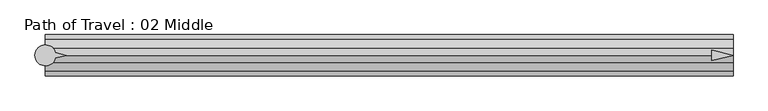
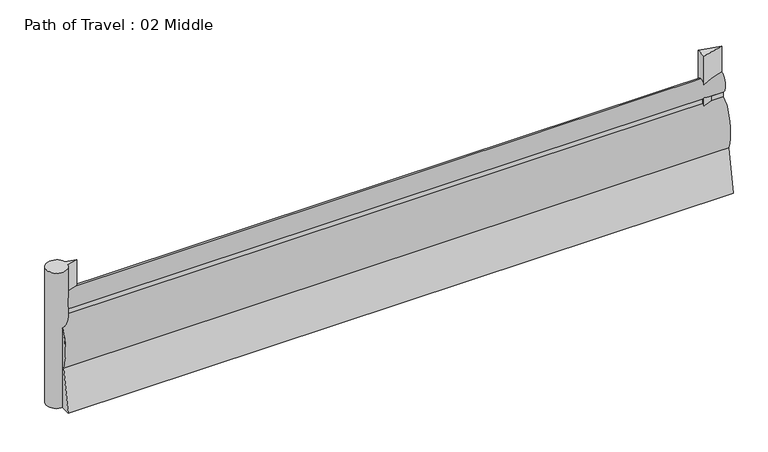
"""IFC4 building model written with IfcOpenShell, lengths in millimetres: proxy geometry, Path of Travel : 02 Middle."""

from ifc_helpers import new_model, si_unit, point, frame, frame_2d, origin, origin_with_axes, place, context, project, spatial, polyline, circle_curve, ellipse_curve, trimmed, segment, composite_curve, outline, extrude, source, transform, mapped, element, save
from ifc_brep_helpers import plane_surface, extruded_surface, advanced_brep


def path_of_travel_02_middle_d07484ce(model_context):
    return source(origin(), model_context, "Body", "SolidModel", [
        advanced_brep(
        [(227.5554837, 0.0, 1727.2), (227.5554837, 42.9018657, 1436.6534209), (227.5554837, 42.9018657, 1363.4763406), (227.5554837, 184.1186263, 643.4144547), (227.5554837, 297.5699544, 0.0), (227.5554837, 145.6574193, 0.0), (227.5554837, 0.0, 584.2), (227.5554837, -145.6574193, 0.0), (227.5554837, -297.5699544, 0.0), (227.5554837, -184.1186263, 643.4144547), (227.5554837, -42.9018657, 1363.4763406), (227.5554837, -42.9018657, 1436.6534209), (10133.5554837, 0.0, 1727.2), (10133.5554837, -42.9018657, 1436.6534209), (10133.5554837, -42.9018657, 1363.4763406), (10133.5554837, -184.1186263, 643.4144547), (10133.5554837, -297.5699544, 0.0), (10133.5554837, -145.6574193, 0.0), (10133.5554837, 0.0, 584.2), (10133.5554837, 145.6574193, 0.0), (10133.5554837, 297.5699544, 0.0), (10133.5554837, 184.1186263, 643.4144547), (10133.5554837, 42.9018657, 1363.4763406), (10133.5554837, 42.9018657, 1436.6534209)],
        [
            (0, 1, ellipse_curve(frame((227.5554837, 0.0, 1574.8), z_axis=(-1.0, 0.0, 0.0), x_axis=(0.0, 0.0, 1.0)), 152.4, 101.6)),
            (1, 2),
            (2, 3, ellipse_curve(frame((227.5554837, 0.0, 914.4), z_axis=(-1.0, 0.0, 0.0), x_axis=(0.0, 0.0, -1.0)), 457.2, 228.6)),
            (3, 4),
            (4, 5),
            (5, 6),
            (6, 7),
            (7, 8),
            (8, 9),
            (9, 10, ellipse_curve(frame((227.5554837, 0.0, 914.4), z_axis=(-1.0, 0.0, 0.0), x_axis=(0.0, 0.0, -1.0)), 457.2, 228.6)),
            (10, 11),
            (11, 0, ellipse_curve(frame((227.5554837, 0.0, 1574.8), z_axis=(-1.0, 0.0, 0.0), x_axis=(0.0, 0.0, 1.0)), 152.4, 101.6)),
            (12, 13, ellipse_curve(frame((10133.5554837, 0.0, 1574.8), z_axis=(1.0, 0.0, 0.0), x_axis=(0.0, 0.0, 1.0)), 152.4, 101.6)),
            (13, 14),
            (14, 15, ellipse_curve(frame((10133.5554837, 0.0, 914.4), z_axis=(1.0, 0.0, 0.0), x_axis=(0.0, 0.0, -1.0)), 457.2, 228.6)),
            (15, 16),
            (16, 17),
            (17, 18),
            (18, 19),
            (19, 20),
            (20, 21),
            (21, 22, ellipse_curve(frame((10133.5554837, 0.0, 914.4), z_axis=(1.0, 0.0, 0.0), x_axis=(0.0, 0.0, -1.0)), 457.2, 228.6)),
            (22, 23),
            (23, 12, ellipse_curve(frame((10133.5554837, 0.0, 1574.8), z_axis=(1.0, 0.0, 0.0), x_axis=(0.0, 0.0, 1.0)), 152.4, 101.6)),
            (0, 12),
            (23, 1),
            (22, 2),
            (21, 3),
            (20, 4),
            (19, 5),
            (18, 6),
            (17, 7),
            (16, 8),
            (15, 9),
            (14, 10),
            (13, 11),
        ],
        [
            plane_surface(frame((227.5554837, 0.0, 0.0), z_axis=(-1.0, 0.0, 0.0), x_axis=(0.0, 0.0, 1.0))),
            plane_surface(frame((10133.5554837, 0.0, 0.0), z_axis=(1.0, 0.0, 0.0), x_axis=(0.0, 0.0, 1.0))),
            extruded_surface(trimmed(ellipse_curve(frame((10133.5554837, 0.0, 1574.8), z_axis=(-1.0, 0.0, 0.0), x_axis=(0.0, 0.0, 1.0)), 152.4, 101.6), [point((10133.5554837, 0.0, 1727.2))], [point((10133.5554837, 42.9018657, 1436.6534209))], True, "CARTESIAN"), (-9906.0, 0.0, 0.0), 9906.0),
            plane_surface(frame((227.5554837, 42.9018657, 1436.6534209), z_axis=(0.0, 1.0, 0.0), x_axis=(1.0, 0.0, 0.0))),
            extruded_surface(trimmed(ellipse_curve(frame((10133.5554837, 0.0, 914.4), z_axis=(-1.0, 0.0, 0.0), x_axis=(0.0, 0.0, -1.0)), 457.2, 228.6), [point((10133.5554837, 42.9018657, 1363.4763406))], [point((10133.5554837, 184.1186263, 643.4144547))], True, "CARTESIAN"), (-9906.0, 0.0, 0.0), 9906.0),
            plane_surface(frame((227.5554837, 184.1186263, 643.4144547), z_axis=(0.0, 0.9848077530122078, 0.1736481776669322), x_axis=(1.0, 0.0, 0.0))),
            plane_surface(frame((227.5554837, 297.5699544, 0.0), z_axis=(0.0, 0.0, -1.0), x_axis=(1.0, 0.0, 0.0))),
            plane_surface(frame((227.5554837, 145.6574193, 0.0), z_axis=(0.0, -0.9702957262760199, -0.2419218955995739), x_axis=(1.0, 0.0, 0.0))),
            plane_surface(frame((227.5554837, 0.0, 584.2), z_axis=(0.0, 0.9702957262759961, -0.24192189559966923), x_axis=(1.0, 0.0, 0.0))),
            plane_surface(frame((227.5554837, -145.6574193, 0.0), z_axis=(0.0, 0.0, -1.0), x_axis=(1.0, 0.0, 0.0))),
            plane_surface(frame((227.5554837, -297.5699544, 0.0), z_axis=(0.0, -0.984807753012208, 0.17364817766693066), x_axis=(1.0, 0.0, 0.0))),
            extruded_surface(trimmed(ellipse_curve(frame((10133.5554837, 0.0, 914.4), z_axis=(-1.0, 0.0, 0.0), x_axis=(0.0, 0.0, -1.0)), 457.2, 228.6), [point((10133.5554837, -184.1186263, 643.4144547))], [point((10133.5554837, -42.9018657, 1363.4763406))], True, "CARTESIAN"), (-9906.0, 0.0, 0.0), 9906.0),
            plane_surface(frame((227.5554837, -42.9018657, 1363.4763406), z_axis=(0.0, -1.0, 0.0), x_axis=(1.0, 0.0, 0.0))),
            extruded_surface(trimmed(ellipse_curve(frame((10133.5554837, 0.0, 1574.8), z_axis=(-1.0, 0.0, 0.0), x_axis=(0.0, 0.0, 1.0)), 152.4, 101.6), [point((10133.5554837, -42.9018657, 1436.6534209))], [point((10133.5554837, 0.0, 1727.2))], True, "CARTESIAN"), (-9906.0, 0.0, 0.0), 9906.0),
        ],
        [
            (0, [[1, 2, 3, 4, 5, 6, 7, 8, 9, 10, 11, 12]]),
            (1, [[13, 14, 15, 16, 17, 18, 19, 20, 21, 22, 23, 24]]),
            (2, [[-1, 25, -24, 26]]),
            (3, [[-2, -26, -23, 27]]),
            (4, [[-3, -27, -22, 28]]),
            (5, [[-4, -28, -21, 29]]),
            (6, [[-5, -29, -20, 30]]),
            (7, [[-6, -30, -19, 31]]),
            (8, [[-7, -31, -18, 32]]),
            (9, [[-8, -32, -17, 33]]),
            (10, [[-9, -33, -16, 34]]),
            (11, [[-10, -34, -15, 35]]),
            (12, [[-11, -35, -14, 36]]),
            (13, [[-12, -36, -13, -25]]),
        ],
    ),
        extrude(outline(polyline([(9827.5503371, 76.2006338), (10133.5554837, 0.0), (9827.5503371, -76.2006338), (9827.5503371, 76.2006338)])), origin_with_axes(), (0.0, 0.0, 1.0), 2129.5973753),
        extrude(outline(composite_curve([segment(polyline([(372.7837828, 39.4440225), (531.182385, 0.0), (372.7837828, -39.4440225)]), True, "CONTINUOUS"), segment(trimmed(circle_curve(frame_2d((227.2200886, 0.0)), 150.8131956), [point((372.7837828, -39.4440225))], [point((372.7837828, 39.4440225))], False, "CARTESIAN"), True, "CONTINUOUS")], self_intersect=False)), origin_with_axes(), (0.0, 0.0, 1.0), 2129.5973753),
    ])


if __name__ == "__main__":
    model = new_model("IFC4")
    model_context = context("Model", 3, world=origin())
    ifc_project = project(units=[si_unit("LENGTHUNIT", "METRE", prefix="MILLI")], contexts=[model_context])
    site = spatial("IfcSite", under=ifc_project)
    building = spatial("IfcBuilding", under=site)
    placement = place(None, origin())
    path_of_travel_02_middle_shape = path_of_travel_02_middle_d07484ce(model_context)
    element("IfcBuildingElementProxy", 1, Name="Path of Travel : 02 Middle", ObjectType="Path of Travel : 02 Middle", at=placement, inside=building, context=model_context, shape_type="MappedRepresentation", body=[
        mapped(path_of_travel_02_middle_shape, transform((0.0, 0.0, 0.0), x_axis=(1.0, 0.0, 0.0), y_axis=(0.0, 1.0, 0.0), z_axis=(0.0, 0.0, 1.0))),
    ])
    save(model, "model.ifc")

# Revit data of these elements
# Type "Path of Travel : 02 Middle"
#   Path of Egress [instance default] = 4' - 0"
#   built-in parameter 1001306 [instance default] = 4 (stored number, unit not read)
#   Dot at Start = no
#   Arrow in Middle = yes
#   Arrow at End = no
#   Egress Path = none
# Element 1 (IfcBuildingElementProxy, "Path of Travel : 02 Middle")
#   Path of Egress = 32' - 6"
#   built-in parameter 1001306 = 32.5 (stored number, unit not read)
